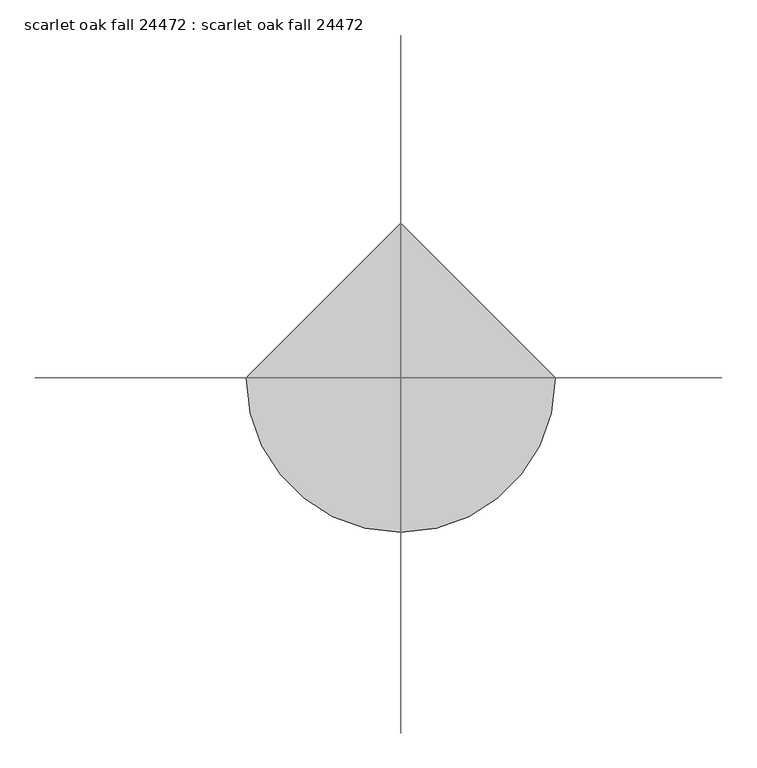
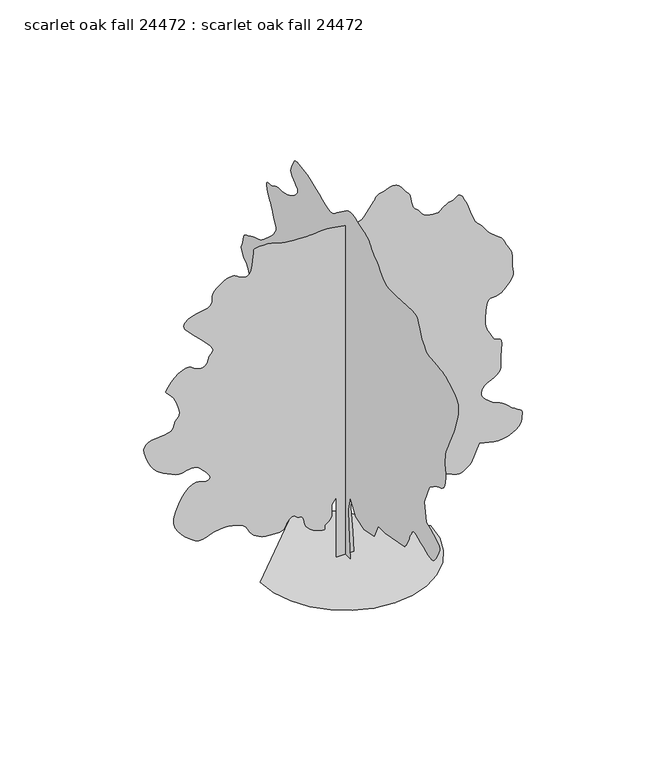
# IFC4 building model written with IfcOpenShell, lengths in millimetres: proxy geometry, scarlet oak fall 24472 : scarlet oak fall 24472.
# Revit data of these elements (continued)
# Type "scarlet oak fall 24472 : scarlet oak fall 24472"
#   built-in parameter 1005195 = "RPC-16-FXGN-QL00-PPP3-E000-ST1L-LVER-AU"
#   Height = 0
